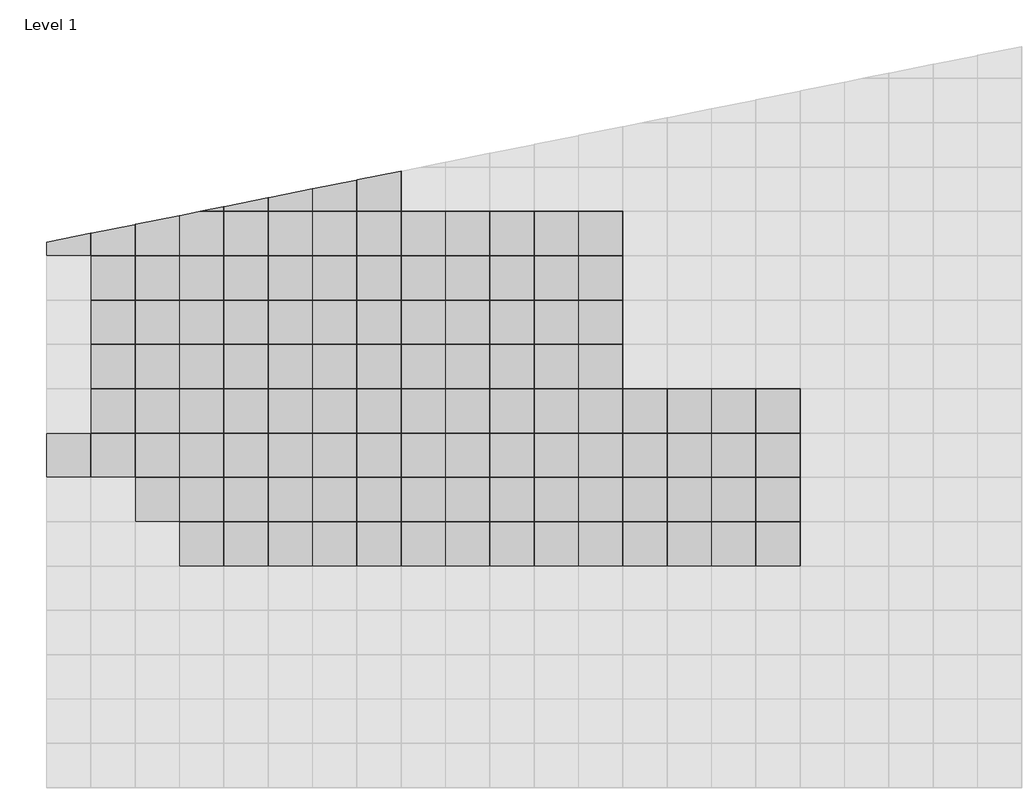
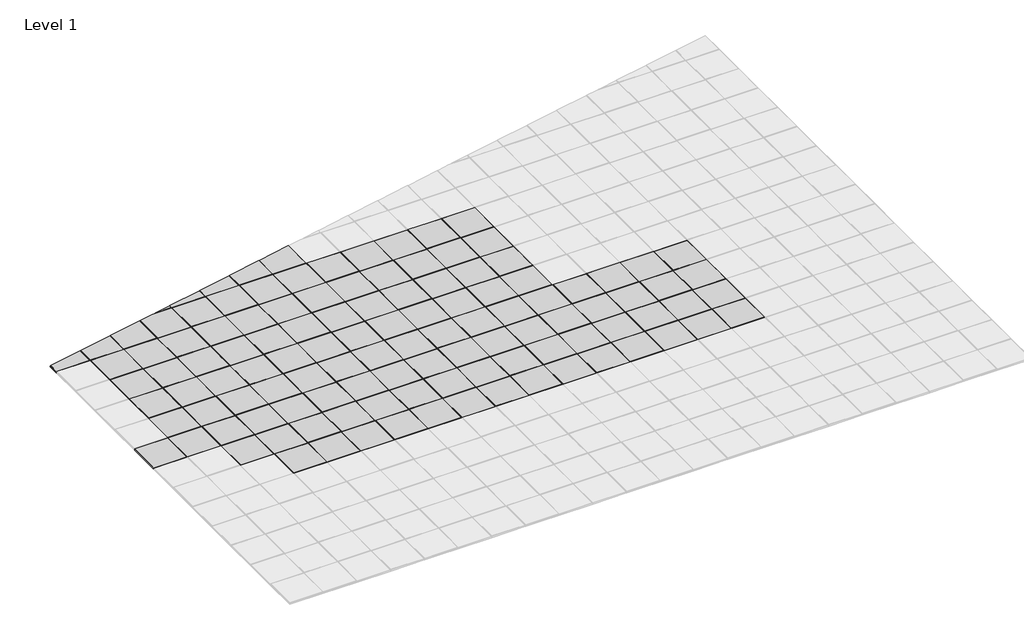
# One storey, part 5 of 18: 116 plates.
"""IFC4 building model written with IfcOpenShell, lengths in millimetres."""

import ifcopenshell
import ifcopenshell.guid

model = None  # the IFC model being written
_history = None  # IfcOwnerHistory: only IFC2X3 demands one
_inside = {}  # id of a spatial element -> (the spatial element, [elements in it])
_under = {}  # id of a project, library or spatial element -> (it, [spatial elements below it])
_declared = {}  # id of a project -> (the project, [libraries it declares])
_typed = {}  # id of a type object -> (the type object, [elements of that type])
_made_of = {}  # id of a material, layer set ... -> (it, [elements and type objects made of it])


def new_model(schema):
    """Start an empty IFC model of exactly this schema.

    Asked for "IFC4X3", IfcOpenShell would pick the latest addendum, in which some entities
    have other attributes; the version numbers below select the first issue.
    IFC2X3 requires an IfcOwnerHistory on every rooted entity: one is made here for all.
    """
    global model, _history
    if schema == "IFC4X3":
        model = ifcopenshell.file(schema_version=(4, 3, 0, 0))
    else:
        model = ifcopenshell.file(schema=schema)
    _inside.clear()
    _under.clear()
    _declared.clear()
    _typed.clear()
    _made_of.clear()
    _history = None
    if model.schema == "IFC2X3":
        org = make("IfcOrganization", Name="unknown")
        user = make(
            "IfcPersonAndOrganization",
            ThePerson=make("IfcPerson", FamilyName="unknown"),
            TheOrganization=org,
        )
        app = make(
            "IfcApplication",
            ApplicationDeveloper=org,
            Version="unknown",
            ApplicationFullName="unknown",
            ApplicationIdentifier="unknown",
        )
        _history = make(
            "IfcOwnerHistory",
            OwningUser=user,
            OwningApplication=app,
            ChangeAction="ADDED",
            CreationDate=0,
        )
    return model


def make(cls, **values):
    """One entity of the class cls with the attributes given. An attribute that is None is left unset."""
    return model.create_entity(
        cls, **{name: value for name, value in values.items() if value is not None}
    )


def rooted(cls, **values):
    """An entity with a GlobalId (a new one), such as an element, a storey or a relation."""
    return make(cls, GlobalId=ifcopenshell.guid.new(), OwnerHistory=_history, **values)


def si_unit(unit_type, name, prefix=None):
    """IfcSIUnit, for example si_unit("LENGTHUNIT", "METRE", prefix="MILLI")."""
    return make("IfcSIUnit", UnitType=unit_type, Prefix=prefix, Name=name)


def assignment(units):
    """IfcUnitAssignment: the units of a project."""
    return None if units is None else make("IfcUnitAssignment", Units=units)


def point(xyz):
    """IfcCartesianPoint."""
    return None if xyz is None else make("IfcCartesianPoint", Coordinates=xyz)


def direction(xyz):
    """IfcDirection."""
    return None if xyz is None else make("IfcDirection", DirectionRatios=xyz)


def frame(location, z_axis=None, x_axis=None):
    """IfcAxis2Placement3D, a coordinate frame: its origin and axes. An axis left out is left unset."""
    return make(
        "IfcAxis2Placement3D",
        Location=point(location),
        Axis=direction(z_axis),
        RefDirection=direction(x_axis),
    )


def origin():
    """The frame at (0, 0, 0) with its axes left unset."""
    return frame((0.0, 0.0, 0.0))


def origin_with_axes():
    """The frame at (0, 0, 0) with the z axis (0, 0, 1) and the x axis (1, 0, 0) written out."""
    return frame((0.0, 0.0, 0.0), z_axis=(0.0, 0.0, 1.0), x_axis=(1.0, 0.0, 0.0))


def place(relative_to, where):
    """IfcLocalPlacement: puts the frame where relative to a parent placement (None: the world)."""
    return make(
        "IfcLocalPlacement", PlacementRelTo=relative_to, RelativePlacement=where
    )


def context(
    kind, dimensions, precision=None, world=None, true_north=None, identifier=None
):
    """IfcGeometricRepresentationContext, for example the 3D "Model" context."""
    return make(
        "IfcGeometricRepresentationContext",
        ContextIdentifier=identifier,
        ContextType=kind,
        CoordinateSpaceDimension=dimensions,
        Precision=precision,
        WorldCoordinateSystem=world,
        TrueNorth=true_north,
    )


def project(units=None, contexts=None):
    """IfcProject with its units and contexts."""
    return rooted(
        "IfcProject",
        Name="project",
        RepresentationContexts=contexts,
        UnitsInContext=assignment(units),
    )


def spatial(cls, under=None, at=None, **own):
    """A site, building, storey or space (cls), placed at a placement, below another one or the project."""
    s = rooted(cls, ObjectPlacement=at, **own)
    if under is not None:
        _under.setdefault(under.id(), (under, []))[1].append(s)
    return s


def polyline(points):
    """IfcPolyline through the points."""
    return make("IfcPolyline", Points=[point(p) for p in points])


def outline(outer, holes=None, kind="AREA"):
    """IfcArbitraryClosedProfileDef: a profile drawn as a closed curve; with holes, ...WithVoids."""
    if holes is None:
        return make("IfcArbitraryClosedProfileDef", ProfileType=kind, OuterCurve=outer)
    return make(
        "IfcArbitraryProfileDefWithVoids",
        ProfileType=kind,
        OuterCurve=outer,
        InnerCurves=holes,
    )


def extrude(swept, where, along, depth):
    """IfcExtrudedAreaSolid: the profile swept, set in the frame where, extruded along a direction by depth."""
    return make(
        "IfcExtrudedAreaSolid",
        SweptArea=swept,
        Position=where,
        ExtrudedDirection=direction(along),
        Depth=depth,
    )


def shape(context_of_items, identifier, shape_type, items):
    """IfcShapeRepresentation: the items that make up one representation, for example the "Body"."""
    return make(
        "IfcShapeRepresentation",
        ContextOfItems=context_of_items,
        RepresentationIdentifier=identifier,
        RepresentationType=shape_type,
        Items=items,
    )


def source(mapping_origin, context_of_items, identifier, shape_type, items):
    """IfcRepresentationMap: a shape defined once, which mapped items show again and again."""
    return make(
        "IfcRepresentationMap",
        MappingOrigin=mapping_origin,
        MappedRepresentation=shape(context_of_items, identifier, shape_type, items),
    )


def transform(
    local_origin,
    x_axis=None,
    y_axis=None,
    z_axis=None,
    scale=None,
    scale2=None,
    scale3=None,
    uniform=True,
):
    """IfcCartesianTransformationOperator3D, or its non-uniform kind. x_axis, y_axis, z_axis: its Axis1, 2, 3."""
    if uniform:
        return make(
            "IfcCartesianTransformationOperator3D",
            Axis1=direction(x_axis),
            Axis2=direction(y_axis),
            LocalOrigin=point(local_origin),
            Scale=scale,
            Axis3=direction(z_axis),
        )
    return make(
        "IfcCartesianTransformationOperator3DnonUniform",
        Axis1=direction(x_axis),
        Axis2=direction(y_axis),
        LocalOrigin=point(local_origin),
        Scale=scale,
        Axis3=direction(z_axis),
        Scale2=scale2,
        Scale3=scale3,
    )


def mapped(mapping_source, mapping_target):
    """IfcMappedItem: shows the shape of a source again, moved by a transform."""
    return make(
        "IfcMappedItem", MappingSource=mapping_source, MappingTarget=mapping_target
    )


def made_of(thing, what):
    """Note that an element or type object is made of a material, layer set ...; save() writes the relation."""
    if what is not None:
        _made_of.setdefault(what.id(), (what, []))[1].append(thing)
    return thing


def element(
    cls,
    number,
    at=None,
    inside=None,
    cuts=None,
    type_object=None,
    material=None,
    context=None,
    identifier="Body",
    shape_type=None,
    held_by="IfcProductDefinitionShape",
    body=None,
    shapes=None,
    **own,
):
    """One element of the class cls, such as IfcWall. Its Tag is "e" and its number.

    at: its placement. inside: the storey or other place that contains it. cuts: it is an
    opening in that element (IfcRelVoidsElement). A single representation is given by context,
    identifier, shape_type and body (its items); several are given by shapes. held_by: the class
    of the entity that holds the representations. save() writes the other relations.
    """
    e = rooted(cls, Tag="e%d" % number, ObjectPlacement=at, **own)
    if body is not None:
        shapes = [shape(context, identifier, shape_type, body)]
    if shapes is not None:
        e.Representation = make(held_by, Representations=shapes)
    if inside is not None:
        _inside.setdefault(inside.id(), (inside, []))[1].append(e)
    if cuts is not None:
        rooted(
            "IfcRelVoidsElement", RelatingBuildingElement=cuts, RelatedOpeningElement=e
        )
    if type_object is not None:
        _typed.setdefault(type_object.id(), (type_object, []))[1].append(e)
    return made_of(e, material)


def aggregate(whole, parts):
    """IfcRelAggregates: a whole, such as a stair, and the parts it consists of."""
    return rooted("IfcRelAggregates", RelatingObject=whole, RelatedObjects=parts)


def save(model, path):
    """Write the relations noted so far, then the file.

    IfcRelAggregates (storeys below a building ...), IfcRelContainedInSpatialStructure (elements
    in a storey), IfcRelDefinesByType, IfcRelAssociatesMaterial and IfcRelDeclares: one each for
    every whole, place, type object, material and project.
    """
    for whole, parts in _under.values():
        aggregate(whole, parts)
    for where, things in _inside.values():
        rooted(
            "IfcRelContainedInSpatialStructure",
            RelatedElements=things,
            RelatingStructure=where,
        )
    for kind, things in _typed.values():
        rooted("IfcRelDefinesByType", RelatedObjects=things, RelatingType=kind)
    for what, things in _made_of.values():
        rooted("IfcRelAssociatesMaterial", RelatedObjects=things, RelatingMaterial=what)
    for by, libraries in _declared.values():
        rooted("IfcRelDeclares", RelatingContext=by, RelatedDefinitions=libraries)
    model.write(path)


def type_1_8eb2385c(model_context):
    return source(origin(), model_context, "Body", "SweptSolid", [
        extrude(outline(polyline([(1000.0, 500.0), (500.0, 500.0), (500.0, 1000.0), (1000.0, 1000.0), (1000.0, 500.0)]), holes=[polyline([(995.0, 995.0), (505.0, 995.0), (505.0, 505.0), (995.0, 505.0), (995.0, 995.0)])]), origin_with_axes(), (0.0, 0.0, 1.0), 18.0),
        extrude(outline(polyline([(505.0, 995.0), (995.0, 995.0), (995.0, 505.0), (505.0, 505.0), (505.0, 995.0)])), origin_with_axes(), (0.0, 0.0, 1.0), 20.0),
    ])


model = new_model("IFC4")

# Units and contexts
model_context = context("Model", 3, world=origin())
ifc_project = project(units=[si_unit("LENGTHUNIT", "METRE", prefix="MILLI")], contexts=[model_context])

# Site, building, storey
site = spatial("IfcSite", under=ifc_project)
building = spatial("IfcBuilding", under=site)
storey = spatial("IfcBuildingStorey", under=building, Name="Level 1", Elevation=0.0)

# Plates
placement = place(None, origin())
element("IfcPlate", 1, ObjectType="00_CPA_tegel : Type 1", at=placement, inside=storey, context=model_context, shape_type="SweptSolid", body=[
    extrude(outline(polyline([(4011.2147669, 18087.7016515), (4501.2147669, 18087.7016515), (4501.2147669, 17597.7016515), (4011.2147669, 17597.7016515), (4011.2147669, 18087.7016515)])), origin_with_axes(), (0.0, 0.0, 1.0), 20.0),
    extrude(outline(polyline([(4506.2147669, 17592.7016515), (4006.2147669, 17592.7016515), (4006.2147669, 18092.7016515), (4506.2147669, 18092.7016515), (4506.2147669, 17592.7016515)]), holes=[polyline([(4501.2147669, 18087.7016515), (4011.2147669, 18087.7016515), (4011.2147669, 17597.7016515), (4501.2147669, 17597.7016515), (4501.2147669, 18087.7016515)])]), origin_with_axes(), (0.0, 0.0, 1.0), 18.0),
])
element("IfcPlate", 2, ObjectType="00_CPA_tegel : Type 1", at=placement, inside=storey, context=model_context, shape_type="SweptSolid", body=[
    extrude(outline(polyline([(4511.2147669, 18087.7016515), (5001.2147669, 18087.7016515), (5001.2147669, 17597.7016515), (4511.2147669, 17597.7016515), (4511.2147669, 18087.7016515)])), origin_with_axes(), (0.0, 0.0, 1.0), 20.0),
    extrude(outline(polyline([(5006.2147669, 17592.7016515), (4506.2147669, 17592.7016515), (4506.2147669, 18092.7016515), (5006.2147669, 18092.7016515), (5006.2147669, 17592.7016515)]), holes=[polyline([(5001.2147669, 18087.7016515), (4511.2147669, 18087.7016515), (4511.2147669, 17597.7016515), (5001.2147669, 17597.7016515), (5001.2147669, 18087.7016515)])]), origin_with_axes(), (0.0, 0.0, 1.0), 18.0),
])
element("IfcPlate", 3, ObjectType="00_CPA_tegel : Type 1", at=placement, inside=storey, context=model_context, shape_type="SweptSolid", body=[
    extrude(outline(polyline([(6511.2147669, 18587.7016515), (7001.2147669, 18587.7016515), (7001.2147669, 18097.7016515), (6511.2147669, 18097.7016515), (6511.2147669, 18587.7016515)])), origin_with_axes(), (0.0, 0.0, 1.0), 20.0),
    extrude(outline(polyline([(7006.2147669, 18092.7016515), (6506.2147669, 18092.7016515), (6506.2147669, 18592.7016515), (7006.2147669, 18592.7016515), (7006.2147669, 18092.7016515)]), holes=[polyline([(7001.2147669, 18587.7016515), (6511.2147669, 18587.7016515), (6511.2147669, 18097.7016515), (7001.2147669, 18097.7016515), (7001.2147669, 18587.7016515)])]), origin_with_axes(), (0.0, 0.0, 1.0), 18.0),
])
element("IfcPlate", 4, ObjectType="00_CPA_tegel : Type 1", at=placement, inside=storey, context=model_context, shape_type="SweptSolid", body=[
    extrude(outline(polyline([(8511.2147669, 19087.7016515), (9001.2147669, 19087.7016515), (9001.2147669, 18597.7016515), (8511.2147669, 18597.7016515), (8511.2147669, 19087.7016515)])), origin_with_axes(), (0.0, 0.0, 1.0), 20.0),
    extrude(outline(polyline([(9006.2147669, 18592.7016515), (8506.2147669, 18592.7016515), (8506.2147669, 19092.7016515), (9006.2147669, 19092.7016515), (9006.2147669, 18592.7016515)]), holes=[polyline([(9001.2147669, 19087.7016515), (8511.2147669, 19087.7016515), (8511.2147669, 18597.7016515), (9001.2147669, 18597.7016515), (9001.2147669, 19087.7016515)])]), origin_with_axes(), (0.0, 0.0, 1.0), 18.0),
])
element("IfcPlate", 5, ObjectType="00_CPA_tegel : Type 1", at=placement, inside=storey, context=model_context, shape_type="SweptSolid", body=[
    extrude(outline(polyline([(4501.2147669, 20097.7016515), (4011.2147669, 20097.7016515), (4011.2147669, 20245.5184604), (4501.2147669, 20343.870772), (4501.2147669, 20097.7016515)])), origin_with_axes(), (0.0, 0.0, 1.0), 20.0),
    extrude(outline(polyline([(4506.2147669, 20092.7016515), (4006.2147669, 20092.7016515), (4006.2147669, 20244.5148654), (4011.2147669, 20245.5184604), (4011.2147669, 20097.7016515), (4501.2147669, 20097.7016515), (4501.2147669, 20343.870772), (4506.2147669, 20344.874367), (4506.2147669, 20092.7016515)])), origin_with_axes(), (0.0, 0.0, 1.0), 18.0),
])
element("IfcPlate", 6, ObjectType="00_CPA_tegel : Type 1", at=placement, inside=storey, context=model_context, shape_type="SweptSolid", body=[
    extrude(outline(polyline([(5001.2147669, 20097.7016515), (4511.2147669, 20097.7016515), (4511.2147669, 20345.8779621), (5001.2147669, 20444.2302737), (5001.2147669, 20097.7016515)])), origin_with_axes(), (0.0, 0.0, 1.0), 20.0),
    extrude(outline(polyline([(5006.2147669, 20092.7016515), (4506.2147669, 20092.7016515), (4506.2147669, 20344.874367), (4511.2147669, 20345.8779621), (4511.2147669, 20097.7016515), (5001.2147669, 20097.7016515), (5001.2147669, 20444.2302737), (5006.2147669, 20445.2338687), (5006.2147669, 20092.7016515)])), origin_with_axes(), (0.0, 0.0, 1.0), 18.0),
])
element("IfcPlate", 7, ObjectType="00_CPA_tegel : Type 1", at=placement, inside=storey, context=model_context, shape_type="SweptSolid", body=[
    extrude(outline(polyline([(5501.2147669, 20097.7016515), (5011.2147669, 20097.7016515), (5011.2147669, 20446.2374637), (5501.2147669, 20544.5897754), (5501.2147669, 20097.7016515)])), origin_with_axes(), (0.0, 0.0, 1.0), 20.0),
    extrude(outline(polyline([(5506.2147669, 20092.7016515), (5006.2147669, 20092.7016515), (5006.2147669, 20445.2338687), (5011.2147669, 20446.2374637), (5011.2147669, 20097.7016515), (5501.2147669, 20097.7016515), (5501.2147669, 20544.5897754), (5506.2147669, 20545.5933704), (5506.2147669, 20092.7016515)])), origin_with_axes(), (0.0, 0.0, 1.0), 18.0),
])
element("IfcPlate", 8, ObjectType="00_CPA_tegel : Type 1", at=placement, inside=storey, context=model_context, shape_type="SweptSolid", body=[
    extrude(outline(polyline([(6001.2147669, 20097.7016515), (5511.2147669, 20097.7016515), (5511.2147669, 20546.5969654), (5716.0019838, 20587.7016515), (6001.2147669, 20587.7016515), (6001.2147669, 20097.7016515)])), origin_with_axes(), (0.0, 0.0, 1.0), 20.0),
    extrude(outline(polyline([(6006.2147669, 20092.7016515), (5506.2147669, 20092.7016515), (5506.2147669, 20545.5933704), (5511.2147669, 20546.5969654), (5511.2147669, 20097.7016515), (6001.2147669, 20097.7016515), (6001.2147669, 20587.7016515), (5716.0019838, 20587.7016515), (5740.9124303, 20592.7016515), (6006.2147669, 20592.7016515), (6006.2147669, 20092.7016515)])), origin_with_axes(), (0.0, 0.0, 1.0), 18.0),
])
element("IfcPlate", 9, ObjectType="00_CPA_tegel : Type 1", at=placement, inside=storey, context=model_context, shape_type="SweptSolid", body=[
    extrude(outline(polyline([(6001.2147669, 20597.7016515), (5765.8228768, 20597.7016515), (6001.2147669, 20644.9492771), (6001.2147669, 20597.7016515)])), origin_with_axes(), (0.0, 0.0, 1.0), 20.0),
    extrude(outline(polyline([(6006.2147669, 20592.7016515), (5740.9124303, 20592.7016515), (5765.8228768, 20597.7016515), (6001.2147669, 20597.7016515), (6001.2147669, 20644.9492771), (6006.2147669, 20645.9528721), (6006.2147669, 20592.7016515)])), origin_with_axes(), (0.0, 0.0, 1.0), 18.0),
])
element("IfcPlate", 10, ObjectType="00_CPA_tegel : Type 1", at=placement, inside=storey, context=model_context, shape_type="SweptSolid", body=[
    extrude(outline(polyline([(6501.2147669, 20597.7016515), (6011.2147669, 20597.7016515), (6011.2147669, 20646.9564671), (6501.2147669, 20745.3087788), (6501.2147669, 20597.7016515)])), origin_with_axes(), (0.0, 0.0, 1.0), 20.0),
    extrude(outline(polyline([(6506.2147669, 20592.7016515), (6006.2147669, 20592.7016515), (6006.2147669, 20645.9528721), (6011.2147669, 20646.9564671), (6011.2147669, 20597.7016515), (6501.2147669, 20597.7016515), (6501.2147669, 20745.3087788), (6506.2147669, 20746.3123738), (6506.2147669, 20592.7016515)])), origin_with_axes(), (0.0, 0.0, 1.0), 18.0),
])
element("IfcPlate", 11, ObjectType="00_CPA_tegel : Type 1", at=placement, inside=storey, context=model_context, shape_type="SweptSolid", body=[
    extrude(outline(polyline([(7001.2147669, 20597.7016515), (6511.2147669, 20597.7016515), (6511.2147669, 20747.3159688), (7001.2147669, 20845.6682804), (7001.2147669, 20597.7016515)])), origin_with_axes(), (0.0, 0.0, 1.0), 20.0),
    extrude(outline(polyline([(7006.2147669, 20592.7016515), (6506.2147669, 20592.7016515), (6506.2147669, 20746.3123738), (6511.2147669, 20747.3159688), (6511.2147669, 20597.7016515), (7001.2147669, 20597.7016515), (7001.2147669, 20845.6682804), (7006.2147669, 20846.6718755), (7006.2147669, 20592.7016515)])), origin_with_axes(), (0.0, 0.0, 1.0), 18.0),
])
element("IfcPlate", 12, ObjectType="00_CPA_tegel : Type 1", at=placement, inside=storey, context=model_context, shape_type="SweptSolid", body=[
    extrude(outline(polyline([(7501.2147669, 20597.7016515), (7011.2147669, 20597.7016515), (7011.2147669, 20847.6754705), (7501.2147669, 20946.0277821), (7501.2147669, 20597.7016515)])), origin_with_axes(), (0.0, 0.0, 1.0), 20.0),
    extrude(outline(polyline([(7506.2147669, 20592.7016515), (7006.2147669, 20592.7016515), (7006.2147669, 20846.6718755), (7011.2147669, 20847.6754705), (7011.2147669, 20597.7016515), (7501.2147669, 20597.7016515), (7501.2147669, 20946.0277821), (7506.2147669, 20947.0313772), (7506.2147669, 20592.7016515)])), origin_with_axes(), (0.0, 0.0, 1.0), 18.0),
])
element("IfcPlate", 13, ObjectType="00_CPA_tegel : Type 1", at=placement, inside=storey, context=model_context, shape_type="SweptSolid", body=[
    extrude(outline(polyline([(8001.2147669, 20597.7016515), (7511.2147669, 20597.7016515), (7511.2147669, 20948.0349722), (8001.2147669, 21046.3872838), (8001.2147669, 20597.7016515)])), origin_with_axes(), (0.0, 0.0, 1.0), 20.0),
    extrude(outline(polyline([(8006.2147669, 20592.7016515), (7506.2147669, 20592.7016515), (7506.2147669, 20947.0313772), (7511.2147669, 20948.0349722), (7511.2147669, 20597.7016515), (8001.2147669, 20597.7016515), (8001.2147669, 21046.3872838), (8006.2147669, 21047.3908788), (8006.2147669, 20592.7016515)])), origin_with_axes(), (0.0, 0.0, 1.0), 18.0),
])
type_1_shape = type_1_8eb2385c(model_context)
element("IfcPlate", 14, ObjectType="00_CPA_tegel : Type 1", at=placement, inside=storey, context=model_context, shape_type="MappedRepresentation", body=[
    mapped(type_1_shape, transform((9006.2147669, 16092.7016515, 0.0), x_axis=(1.0000000000000002, 0.0, 0.0), y_axis=(0.0, 1.0000000000000002, 0.0), z_axis=(0.0, 0.0, 1.0))),
])
element("IfcPlate", 15, ObjectType="00_CPA_tegel : Type 1", at=placement, inside=storey, context=model_context, shape_type="MappedRepresentation", body=[
    mapped(type_1_shape, transform((9506.2147669, 16092.7016515, 0.0), x_axis=(1.0000000000000002, 0.0, 0.0), y_axis=(0.0, 1.0000000000000002, 0.0), z_axis=(0.0, 0.0, 1.0))),
])
element("IfcPlate", 16, ObjectType="00_CPA_tegel : Type 1", at=placement, inside=storey, context=model_context, shape_type="MappedRepresentation", body=[
    mapped(type_1_shape, transform((6006.2147669, 16092.7016515, 0.0), x_axis=(1.0000000000000002, 0.0, 0.0), y_axis=(0.0, 1.0000000000000002, 0.0), z_axis=(0.0, 0.0, 1.0))),
])
element("IfcPlate", 17, ObjectType="00_CPA_tegel : Type 1", at=placement, inside=storey, context=model_context, shape_type="MappedRepresentation", body=[
    mapped(type_1_shape, transform((6506.2147669, 16092.7016515, 0.0), x_axis=(1.0000000000000002, 0.0, 0.0), y_axis=(0.0, 1.0000000000000002, 0.0), z_axis=(0.0, 0.0, 1.0))),
])
element("IfcPlate", 18, ObjectType="00_CPA_tegel : Type 1", at=placement, inside=storey, context=model_context, shape_type="MappedRepresentation", body=[
    mapped(type_1_shape, transform((7006.2147669, 16092.7016515, 0.0), x_axis=(1.0000000000000002, 0.0, 0.0), y_axis=(0.0, 1.0000000000000002, 0.0), z_axis=(0.0, 0.0, 1.0))),
])
element("IfcPlate", 19, ObjectType="00_CPA_tegel : Type 1", at=placement, inside=storey, context=model_context, shape_type="MappedRepresentation", body=[
    mapped(type_1_shape, transform((7506.2147669, 16092.7016515, 0.0), x_axis=(1.0000000000000002, 0.0, 0.0), y_axis=(0.0, 1.0000000000000002, 0.0), z_axis=(0.0, 0.0, 1.0))),
])
element("IfcPlate", 20, ObjectType="00_CPA_tegel : Type 1", at=placement, inside=storey, context=model_context, shape_type="MappedRepresentation", body=[
    mapped(type_1_shape, transform((8006.2147669, 16092.7016515, 0.0), x_axis=(1.0000000000000002, 0.0, 0.0), y_axis=(0.0, 1.0000000000000002, 0.0), z_axis=(0.0, 0.0, 1.0))),
])
element("IfcPlate", 21, ObjectType="00_CPA_tegel : Type 1", at=placement, inside=storey, context=model_context, shape_type="MappedRepresentation", body=[
    mapped(type_1_shape, transform((8506.2147669, 16092.7016515, 0.0), x_axis=(1.0000000000000002, 0.0, 0.0), y_axis=(0.0, 1.0000000000000002, 0.0), z_axis=(0.0, 0.0, 1.0))),
])
element("IfcPlate", 22, ObjectType="00_CPA_tegel : Type 1", at=placement, inside=storey, context=model_context, shape_type="MappedRepresentation", body=[
    mapped(type_1_shape, transform((8506.2147669, 16592.7016515, 0.0), x_axis=(1.0000000000000002, 0.0, 0.0), y_axis=(0.0, 1.0000000000000002, 0.0), z_axis=(0.0, 0.0, 1.0))),
])
element("IfcPlate", 23, ObjectType="00_CPA_tegel : Type 1", at=placement, inside=storey, context=model_context, shape_type="MappedRepresentation", body=[
    mapped(type_1_shape, transform((9006.2147669, 16592.7016515, 0.0), x_axis=(1.0000000000000002, 0.0, 0.0), y_axis=(0.0, 1.0000000000000002, 0.0), z_axis=(0.0, 0.0, 1.0))),
])
element("IfcPlate", 24, ObjectType="00_CPA_tegel : Type 1", at=placement, inside=storey, context=model_context, shape_type="MappedRepresentation", body=[
    mapped(type_1_shape, transform((9506.2147669, 16592.7016515, 0.0), x_axis=(1.0000000000000002, 0.0, 0.0), y_axis=(0.0, 1.0000000000000002, 0.0), z_axis=(0.0, 0.0, 1.0))),
])
element("IfcPlate", 25, ObjectType="00_CPA_tegel : Type 1", at=placement, inside=storey, context=model_context, shape_type="MappedRepresentation", body=[
    mapped(type_1_shape, transform((5506.2147669, 16092.7016515, 0.0), x_axis=(1.0000000000000002, 0.0, 0.0), y_axis=(0.0, 1.0000000000000002, 0.0), z_axis=(0.0, 0.0, 1.0))),
])
element("IfcPlate", 26, ObjectType="00_CPA_tegel : Type 1", at=placement, inside=storey, context=model_context, shape_type="MappedRepresentation", body=[
    mapped(type_1_shape, transform((7506.2147669, 16592.7016515, 0.0), x_axis=(1.0000000000000002, 0.0, 0.0), y_axis=(0.0, 1.0000000000000002, 0.0), z_axis=(0.0, 0.0, 1.0))),
])
element("IfcPlate", 27, ObjectType="00_CPA_tegel : Type 1", at=placement, inside=storey, context=model_context, shape_type="MappedRepresentation", body=[
    mapped(type_1_shape, transform((8006.2147669, 16592.7016515, 0.0), x_axis=(1.0000000000000002, 0.0, 0.0), y_axis=(0.0, 1.0000000000000002, 0.0), z_axis=(0.0, 0.0, 1.0))),
])
element("IfcPlate", 28, ObjectType="00_CPA_tegel : Type 1", at=placement, inside=storey, context=model_context, shape_type="MappedRepresentation", body=[
    mapped(type_1_shape, transform((10006.2147669, 16592.7016515, 0.0), x_axis=(1.0000000000000002, 0.0, 0.0), y_axis=(0.0, 1.0000000000000002, 0.0), z_axis=(0.0, 0.0, 1.0))),
])
element("IfcPlate", 29, ObjectType="00_CPA_tegel : Type 1", at=placement, inside=storey, context=model_context, shape_type="MappedRepresentation", body=[
    mapped(type_1_shape, transform((10006.2147669, 17092.7016515, 0.0), x_axis=(1.0000000000000002, 0.0, 0.0), y_axis=(0.0, 1.0000000000000002, 0.0), z_axis=(0.0, 0.0, 1.0))),
])
element("IfcPlate", 30, ObjectType="00_CPA_tegel : Type 1", at=placement, inside=storey, context=model_context, shape_type="MappedRepresentation", body=[
    mapped(type_1_shape, transform((5006.2147669, 16092.7016515, 0.0), x_axis=(1.0000000000000002, 0.0, 0.0), y_axis=(0.0, 1.0000000000000002, 0.0), z_axis=(0.0, 0.0, 1.0))),
])
element("IfcPlate", 31, ObjectType="00_CPA_tegel : Type 1", at=placement, inside=storey, context=model_context, shape_type="MappedRepresentation", body=[
    mapped(type_1_shape, transform((10006.2147669, 16092.7016515, 0.0), x_axis=(1.0000000000000002, 0.0, 0.0), y_axis=(0.0, 1.0000000000000002, 0.0), z_axis=(0.0, 0.0, 1.0))),
])
element("IfcPlate", 32, ObjectType="00_CPA_tegel : Type 1", at=placement, inside=storey, context=model_context, shape_type="MappedRepresentation", body=[
    mapped(type_1_shape, transform((9506.2147669, 17092.7016515, 0.0), x_axis=(1.0000000000000002, 0.0, 0.0), y_axis=(0.0, 1.0000000000000002, 0.0), z_axis=(0.0, 0.0, 1.0))),
])
element("IfcPlate", 33, ObjectType="00_CPA_tegel : Type 1", at=placement, inside=storey, context=model_context, shape_type="MappedRepresentation", body=[
    mapped(type_1_shape, transform((6006.2147669, 16592.7016515, 0.0), x_axis=(1.0000000000000002, 0.0, 0.0), y_axis=(0.0, 1.0000000000000002, 0.0), z_axis=(0.0, 0.0, 1.0))),
])
element("IfcPlate", 34, ObjectType="00_CPA_tegel : Type 1", at=placement, inside=storey, context=model_context, shape_type="MappedRepresentation", body=[
    mapped(type_1_shape, transform((6506.2147669, 16592.7016515, 0.0), x_axis=(1.0000000000000002, 0.0, 0.0), y_axis=(0.0, 1.0000000000000002, 0.0), z_axis=(0.0, 0.0, 1.0))),
])
element("IfcPlate", 35, ObjectType="00_CPA_tegel : Type 1", at=placement, inside=storey, context=model_context, shape_type="MappedRepresentation", body=[
    mapped(type_1_shape, transform((7006.2147669, 16592.7016515, 0.0), x_axis=(1.0000000000000002, 0.0, 0.0), y_axis=(0.0, 1.0000000000000002, 0.0), z_axis=(0.0, 0.0, 1.0))),
])
element("IfcPlate", 36, ObjectType="00_CPA_tegel : Type 1", at=placement, inside=storey, context=model_context, shape_type="MappedRepresentation", body=[
    mapped(type_1_shape, transform((8006.2147669, 17092.7016515, 0.0), x_axis=(1.0000000000000002, 0.0, 0.0), y_axis=(0.0, 1.0000000000000002, 0.0), z_axis=(0.0, 0.0, 1.0))),
])
element("IfcPlate", 37, ObjectType="00_CPA_tegel : Type 1", at=placement, inside=storey, context=model_context, shape_type="MappedRepresentation", body=[
    mapped(type_1_shape, transform((8506.2147669, 17092.7016515, 0.0), x_axis=(1.0000000000000002, 0.0, 0.0), y_axis=(0.0, 1.0000000000000002, 0.0), z_axis=(0.0, 0.0, 1.0))),
])
element("IfcPlate", 38, ObjectType="00_CPA_tegel : Type 1", at=placement, inside=storey, context=model_context, shape_type="MappedRepresentation", body=[
    mapped(type_1_shape, transform((9006.2147669, 17092.7016515, 0.0), x_axis=(1.0000000000000002, 0.0, 0.0), y_axis=(0.0, 1.0000000000000002, 0.0), z_axis=(0.0, 0.0, 1.0))),
])
element("IfcPlate", 39, ObjectType="00_CPA_tegel : Type 1", at=placement, inside=storey, context=model_context, shape_type="MappedRepresentation", body=[
    mapped(type_1_shape, transform((10506.2147669, 17092.7016515, 0.0), x_axis=(1.0000000000000002, 0.0, 0.0), y_axis=(0.0, 1.0000000000000002, 0.0), z_axis=(0.0, 0.0, 1.0))),
])
element("IfcPlate", 40, ObjectType="00_CPA_tegel : Type 1", at=placement, inside=storey, context=model_context, shape_type="MappedRepresentation", body=[
    mapped(type_1_shape, transform((10506.2147669, 17592.7016515, 0.0), x_axis=(1.0000000000000002, 0.0, 0.0), y_axis=(0.0, 1.0000000000000002, 0.0), z_axis=(0.0, 0.0, 1.0))),
])
element("IfcPlate", 41, ObjectType="00_CPA_tegel : Type 1", at=placement, inside=storey, context=model_context, shape_type="MappedRepresentation", body=[
    mapped(type_1_shape, transform((10506.2147669, 16092.7016515, 0.0), x_axis=(1.0000000000000002, 0.0, 0.0), y_axis=(0.0, 1.0000000000000002, 0.0), z_axis=(0.0, 0.0, 1.0))),
])
element("IfcPlate", 42, ObjectType="00_CPA_tegel : Type 1", at=placement, inside=storey, context=model_context, shape_type="MappedRepresentation", body=[
    mapped(type_1_shape, transform((4506.2147669, 16592.7016515, 0.0), x_axis=(1.0000000000000002, 0.0, 0.0), y_axis=(0.0, 1.0000000000000002, 0.0), z_axis=(0.0, 0.0, 1.0))),
])
element("IfcPlate", 43, ObjectType="00_CPA_tegel : Type 1", at=placement, inside=storey, context=model_context, shape_type="MappedRepresentation", body=[
    mapped(type_1_shape, transform((5006.2147669, 16592.7016515, 0.0), x_axis=(1.0000000000000002, 0.0, 0.0), y_axis=(0.0, 1.0000000000000002, 0.0), z_axis=(0.0, 0.0, 1.0))),
])
element("IfcPlate", 44, ObjectType="00_CPA_tegel : Type 1", at=placement, inside=storey, context=model_context, shape_type="MappedRepresentation", body=[
    mapped(type_1_shape, transform((5506.2147669, 16592.7016515, 0.0), x_axis=(1.0000000000000002, 0.0, 0.0), y_axis=(0.0, 1.0000000000000002, 0.0), z_axis=(0.0, 0.0, 1.0))),
])
element("IfcPlate", 45, ObjectType="00_CPA_tegel : Type 1", at=placement, inside=storey, context=model_context, shape_type="MappedRepresentation", body=[
    mapped(type_1_shape, transform((10506.2147669, 16592.7016515, 0.0), x_axis=(1.0000000000000002, 0.0, 0.0), y_axis=(0.0, 1.0000000000000002, 0.0), z_axis=(0.0, 0.0, 1.0))),
])
element("IfcPlate", 46, ObjectType="00_CPA_tegel : Type 1", at=placement, inside=storey, context=model_context, shape_type="MappedRepresentation", body=[
    mapped(type_1_shape, transform((11006.2147669, 16592.7016515, 0.0), x_axis=(1.0000000000000002, 0.0, 0.0), y_axis=(0.0, 1.0000000000000002, 0.0), z_axis=(0.0, 0.0, 1.0))),
])
element("IfcPlate", 47, ObjectType="00_CPA_tegel : Type 1", at=placement, inside=storey, context=model_context, shape_type="MappedRepresentation", body=[
    mapped(type_1_shape, transform((5506.2147669, 17092.7016515, 0.0), x_axis=(1.0000000000000002, 0.0, 0.0), y_axis=(0.0, 1.0000000000000002, 0.0), z_axis=(0.0, 0.0, 1.0))),
])
element("IfcPlate", 48, ObjectType="00_CPA_tegel : Type 1", at=placement, inside=storey, context=model_context, shape_type="MappedRepresentation", body=[
    mapped(type_1_shape, transform((6006.2147669, 17092.7016515, 0.0), x_axis=(1.0000000000000002, 0.0, 0.0), y_axis=(0.0, 1.0000000000000002, 0.0), z_axis=(0.0, 0.0, 1.0))),
])
element("IfcPlate", 49, ObjectType="00_CPA_tegel : Type 1", at=placement, inside=storey, context=model_context, shape_type="MappedRepresentation", body=[
    mapped(type_1_shape, transform((6506.2147669, 17092.7016515, 0.0), x_axis=(1.0000000000000002, 0.0, 0.0), y_axis=(0.0, 1.0000000000000002, 0.0), z_axis=(0.0, 0.0, 1.0))),
])
element("IfcPlate", 50, ObjectType="00_CPA_tegel : Type 1", at=placement, inside=storey, context=model_context, shape_type="MappedRepresentation", body=[
    mapped(type_1_shape, transform((7006.2147669, 17092.7016515, 0.0), x_axis=(1.0000000000000002, 0.0, 0.0), y_axis=(0.0, 1.0000000000000002, 0.0), z_axis=(0.0, 0.0, 1.0))),
])
element("IfcPlate", 51, ObjectType="00_CPA_tegel : Type 1", at=placement, inside=storey, context=model_context, shape_type="MappedRepresentation", body=[
    mapped(type_1_shape, transform((7506.2147669, 17092.7016515, 0.0), x_axis=(1.0000000000000002, 0.0, 0.0), y_axis=(0.0, 1.0000000000000002, 0.0), z_axis=(0.0, 0.0, 1.0))),
])
element("IfcPlate", 52, ObjectType="00_CPA_tegel : Type 1", at=placement, inside=storey, context=model_context, shape_type="MappedRepresentation", body=[
    mapped(type_1_shape, transform((11006.2147669, 17092.7016515, 0.0), x_axis=(1.0000000000000002, 0.0, 0.0), y_axis=(0.0, 1.0000000000000002, 0.0), z_axis=(0.0, 0.0, 1.0))),
])
element("IfcPlate", 53, ObjectType="00_CPA_tegel : Type 1", at=placement, inside=storey, context=model_context, shape_type="MappedRepresentation", body=[
    mapped(type_1_shape, transform((7506.2147669, 17592.7016515, 0.0), x_axis=(1.0000000000000002, 0.0, 0.0), y_axis=(0.0, 1.0000000000000002, 0.0), z_axis=(0.0, 0.0, 1.0))),
])
element("IfcPlate", 54, ObjectType="00_CPA_tegel : Type 1", at=placement, inside=storey, context=model_context, shape_type="MappedRepresentation", body=[
    mapped(type_1_shape, transform((8006.2147669, 17592.7016515, 0.0), x_axis=(1.0000000000000002, 0.0, 0.0), y_axis=(0.0, 1.0000000000000002, 0.0), z_axis=(0.0, 0.0, 1.0))),
])
element("IfcPlate", 55, ObjectType="00_CPA_tegel : Type 1", at=placement, inside=storey, context=model_context, shape_type="MappedRepresentation", body=[
    mapped(type_1_shape, transform((8506.2147669, 17592.7016515, 0.0), x_axis=(1.0000000000000002, 0.0, 0.0), y_axis=(0.0, 1.0000000000000002, 0.0), z_axis=(0.0, 0.0, 1.0))),
])
element("IfcPlate", 56, ObjectType="00_CPA_tegel : Type 1", at=placement, inside=storey, context=model_context, shape_type="MappedRepresentation", body=[
    mapped(type_1_shape, transform((9006.2147669, 17592.7016515, 0.0), x_axis=(1.0000000000000002, 0.0, 0.0), y_axis=(0.0, 1.0000000000000002, 0.0), z_axis=(0.0, 0.0, 1.0))),
])
element("IfcPlate", 57, ObjectType="00_CPA_tegel : Type 1", at=placement, inside=storey, context=model_context, shape_type="MappedRepresentation", body=[
    mapped(type_1_shape, transform((9506.2147669, 17592.7016515, 0.0), x_axis=(1.0000000000000002, 0.0, 0.0), y_axis=(0.0, 1.0000000000000002, 0.0), z_axis=(0.0, 0.0, 1.0))),
])
element("IfcPlate", 58, ObjectType="00_CPA_tegel : Type 1", at=placement, inside=storey, context=model_context, shape_type="MappedRepresentation", body=[
    mapped(type_1_shape, transform((10006.2147669, 17592.7016515, 0.0), x_axis=(1.0000000000000002, 0.0, 0.0), y_axis=(0.0, 1.0000000000000002, 0.0), z_axis=(0.0, 0.0, 1.0))),
])
element("IfcPlate", 59, ObjectType="00_CPA_tegel : Type 1", at=placement, inside=storey, context=model_context, shape_type="MappedRepresentation", body=[
    mapped(type_1_shape, transform((11006.2147669, 17592.7016515, 0.0), x_axis=(1.0000000000000002, 0.0, 0.0), y_axis=(0.0, 1.0000000000000002, 0.0), z_axis=(0.0, 0.0, 1.0))),
])
element("IfcPlate", 60, ObjectType="00_CPA_tegel : Type 1", at=placement, inside=storey, context=model_context, shape_type="MappedRepresentation", body=[
    mapped(type_1_shape, transform((11006.2147669, 16092.7016515, 0.0), x_axis=(1.0000000000000002, 0.0, 0.0), y_axis=(0.0, 1.0000000000000002, 0.0), z_axis=(0.0, 0.0, 1.0))),
])
element("IfcPlate", 61, ObjectType="00_CPA_tegel : Type 1", at=placement, inside=storey, context=model_context, shape_type="MappedRepresentation", body=[
    mapped(type_1_shape, transform((11506.2147669, 16092.7016515, 0.0), x_axis=(1.0000000000000002, 0.0, 0.0), y_axis=(0.0, 1.0000000000000002, 0.0), z_axis=(0.0, 0.0, 1.0))),
])
element("IfcPlate", 62, ObjectType="00_CPA_tegel : Type 1", at=placement, inside=storey, context=model_context, shape_type="MappedRepresentation", body=[
    mapped(type_1_shape, transform((11506.2147669, 16592.7016515, 0.0), x_axis=(1.0000000000000002, 0.0, 0.0), y_axis=(0.0, 1.0000000000000002, 0.0), z_axis=(0.0, 0.0, 1.0))),
])
element("IfcPlate", 63, ObjectType="00_CPA_tegel : Type 1", at=placement, inside=storey, context=model_context, shape_type="MappedRepresentation", body=[
    mapped(type_1_shape, transform((4506.2147669, 17092.7016515, 0.0), x_axis=(1.0000000000000002, 0.0, 0.0), y_axis=(0.0, 1.0000000000000002, 0.0), z_axis=(0.0, 0.0, 1.0))),
])
element("IfcPlate", 64, ObjectType="00_CPA_tegel : Type 1", at=placement, inside=storey, context=model_context, shape_type="MappedRepresentation", body=[
    mapped(type_1_shape, transform((5006.2147669, 17092.7016515, 0.0), x_axis=(1.0000000000000002, 0.0, 0.0), y_axis=(0.0, 1.0000000000000002, 0.0), z_axis=(0.0, 0.0, 1.0))),
])
element("IfcPlate", 65, ObjectType="00_CPA_tegel : Type 1", at=placement, inside=storey, context=model_context, shape_type="MappedRepresentation", body=[
    mapped(type_1_shape, transform((11506.2147669, 17092.7016515, 0.0), x_axis=(1.0000000000000002, 0.0, 0.0), y_axis=(0.0, 1.0000000000000002, 0.0), z_axis=(0.0, 0.0, 1.0))),
])
element("IfcPlate", 66, ObjectType="00_CPA_tegel : Type 1", at=placement, inside=storey, context=model_context, shape_type="MappedRepresentation", body=[
    mapped(type_1_shape, transform((4006.2147669, 17592.7016515, 0.0), x_axis=(1.0000000000000002, 0.0, 0.0), y_axis=(0.0, 1.0000000000000002, 0.0), z_axis=(0.0, 0.0, 1.0))),
])
element("IfcPlate", 67, ObjectType="00_CPA_tegel : Type 1", at=placement, inside=storey, context=model_context, shape_type="MappedRepresentation", body=[
    mapped(type_1_shape, transform((4506.2147669, 17592.7016515, 0.0), x_axis=(1.0000000000000002, 0.0, 0.0), y_axis=(0.0, 1.0000000000000002, 0.0), z_axis=(0.0, 0.0, 1.0))),
])
element("IfcPlate", 68, ObjectType="00_CPA_tegel : Type 1", at=placement, inside=storey, context=model_context, shape_type="MappedRepresentation", body=[
    mapped(type_1_shape, transform((5006.2147669, 17592.7016515, 0.0), x_axis=(1.0000000000000002, 0.0, 0.0), y_axis=(0.0, 1.0000000000000002, 0.0), z_axis=(0.0, 0.0, 1.0))),
])
element("IfcPlate", 69, ObjectType="00_CPA_tegel : Type 1", at=placement, inside=storey, context=model_context, shape_type="MappedRepresentation", body=[
    mapped(type_1_shape, transform((5506.2147669, 17592.7016515, 0.0), x_axis=(1.0000000000000002, 0.0, 0.0), y_axis=(0.0, 1.0000000000000002, 0.0), z_axis=(0.0, 0.0, 1.0))),
])
element("IfcPlate", 70, ObjectType="00_CPA_tegel : Type 1", at=placement, inside=storey, context=model_context, shape_type="MappedRepresentation", body=[
    mapped(type_1_shape, transform((6506.2147669, 17592.7016515, 0.0), x_axis=(1.0000000000000002, 0.0, 0.0), y_axis=(0.0, 1.0000000000000002, 0.0), z_axis=(0.0, 0.0, 1.0))),
])
element("IfcPlate", 71, ObjectType="00_CPA_tegel : Type 1", at=placement, inside=storey, context=model_context, shape_type="MappedRepresentation", body=[
    mapped(type_1_shape, transform((7006.2147669, 17592.7016515, 0.0), x_axis=(1.0000000000000002, 0.0, 0.0), y_axis=(0.0, 1.0000000000000002, 0.0), z_axis=(0.0, 0.0, 1.0))),
])
element("IfcPlate", 72, ObjectType="00_CPA_tegel : Type 1", at=placement, inside=storey, context=model_context, shape_type="MappedRepresentation", body=[
    mapped(type_1_shape, transform((11506.2147669, 17592.7016515, 0.0), x_axis=(1.0000000000000002, 0.0, 0.0), y_axis=(0.0, 1.0000000000000002, 0.0), z_axis=(0.0, 0.0, 1.0))),
])
element("IfcPlate", 73, ObjectType="00_CPA_tegel : Type 1", at=placement, inside=storey, context=model_context, shape_type="MappedRepresentation", body=[
    mapped(type_1_shape, transform((4006.2147669, 18092.7016515, 0.0), x_axis=(1.0000000000000002, 0.0, 0.0), y_axis=(0.0, 1.0000000000000002, 0.0), z_axis=(0.0, 0.0, 1.0))),
])
element("IfcPlate", 74, ObjectType="00_CPA_tegel : Type 1", at=placement, inside=storey, context=model_context, shape_type="MappedRepresentation", body=[
    mapped(type_1_shape, transform((4506.2147669, 18092.7016515, 0.0), x_axis=(1.0000000000000002, 0.0, 0.0), y_axis=(0.0, 1.0000000000000002, 0.0), z_axis=(0.0, 0.0, 1.0))),
])
element("IfcPlate", 75, ObjectType="00_CPA_tegel : Type 1", at=placement, inside=storey, context=model_context, shape_type="MappedRepresentation", body=[
    mapped(type_1_shape, transform((5006.2147669, 18092.7016515, 0.0), x_axis=(1.0000000000000002, 0.0, 0.0), y_axis=(0.0, 1.0000000000000002, 0.0), z_axis=(0.0, 0.0, 1.0))),
])
element("IfcPlate", 76, ObjectType="00_CPA_tegel : Type 1", at=placement, inside=storey, context=model_context, shape_type="MappedRepresentation", body=[
    mapped(type_1_shape, transform((5506.2147669, 18092.7016515, 0.0), x_axis=(1.0000000000000002, 0.0, 0.0), y_axis=(0.0, 1.0000000000000002, 0.0), z_axis=(0.0, 0.0, 1.0))),
])
element("IfcPlate", 77, ObjectType="00_CPA_tegel : Type 1", at=placement, inside=storey, context=model_context, shape_type="MappedRepresentation", body=[
    mapped(type_1_shape, transform((6006.2147669, 18092.7016515, 0.0), x_axis=(1.0000000000000002, 0.0, 0.0), y_axis=(0.0, 1.0000000000000002, 0.0), z_axis=(0.0, 0.0, 1.0))),
])
element("IfcPlate", 78, ObjectType="00_CPA_tegel : Type 1", at=placement, inside=storey, context=model_context, shape_type="MappedRepresentation", body=[
    mapped(type_1_shape, transform((6506.2147669, 18092.7016515, 0.0), x_axis=(1.0000000000000002, 0.0, 0.0), y_axis=(0.0, 1.0000000000000002, 0.0), z_axis=(0.0, 0.0, 1.0))),
])
element("IfcPlate", 79, ObjectType="00_CPA_tegel : Type 1", at=placement, inside=storey, context=model_context, shape_type="MappedRepresentation", body=[
    mapped(type_1_shape, transform((7006.2147669, 18092.7016515, 0.0), x_axis=(1.0000000000000002, 0.0, 0.0), y_axis=(0.0, 1.0000000000000002, 0.0), z_axis=(0.0, 0.0, 1.0))),
])
element("IfcPlate", 80, ObjectType="00_CPA_tegel : Type 1", at=placement, inside=storey, context=model_context, shape_type="MappedRepresentation", body=[
    mapped(type_1_shape, transform((7506.2147669, 18092.7016515, 0.0), x_axis=(1.0000000000000002, 0.0, 0.0), y_axis=(0.0, 1.0000000000000002, 0.0), z_axis=(0.0, 0.0, 1.0))),
])
element("IfcPlate", 81, ObjectType="00_CPA_tegel : Type 1", at=placement, inside=storey, context=model_context, shape_type="MappedRepresentation", body=[
    mapped(type_1_shape, transform((8506.2147669, 18092.7016515, 0.0), x_axis=(1.0000000000000002, 0.0, 0.0), y_axis=(0.0, 1.0000000000000002, 0.0), z_axis=(0.0, 0.0, 1.0))),
])
element("IfcPlate", 82, ObjectType="00_CPA_tegel : Type 1", at=placement, inside=storey, context=model_context, shape_type="MappedRepresentation", body=[
    mapped(type_1_shape, transform((9006.2147669, 18092.7016515, 0.0), x_axis=(1.0000000000000002, 0.0, 0.0), y_axis=(0.0, 1.0000000000000002, 0.0), z_axis=(0.0, 0.0, 1.0))),
])
element("IfcPlate", 83, ObjectType="00_CPA_tegel : Type 1", at=placement, inside=storey, context=model_context, shape_type="MappedRepresentation", body=[
    mapped(type_1_shape, transform((9506.2147669, 18092.7016515, 0.0), x_axis=(1.0000000000000002, 0.0, 0.0), y_axis=(0.0, 1.0000000000000002, 0.0), z_axis=(0.0, 0.0, 1.0))),
])
element("IfcPlate", 84, ObjectType="00_CPA_tegel : Type 1", at=placement, inside=storey, context=model_context, shape_type="MappedRepresentation", body=[
    mapped(type_1_shape, transform((4006.2147669, 18592.7016515, 0.0), x_axis=(1.0000000000000002, 0.0, 0.0), y_axis=(0.0, 1.0000000000000002, 0.0), z_axis=(0.0, 0.0, 1.0))),
])
element("IfcPlate", 85, ObjectType="00_CPA_tegel : Type 1", at=placement, inside=storey, context=model_context, shape_type="MappedRepresentation", body=[
    mapped(type_1_shape, transform((4506.2147669, 18592.7016515, 0.0), x_axis=(1.0000000000000002, 0.0, 0.0), y_axis=(0.0, 1.0000000000000002, 0.0), z_axis=(0.0, 0.0, 1.0))),
])
element("IfcPlate", 86, ObjectType="00_CPA_tegel : Type 1", at=placement, inside=storey, context=model_context, shape_type="MappedRepresentation", body=[
    mapped(type_1_shape, transform((5006.2147669, 18592.7016515, 0.0), x_axis=(1.0000000000000002, 0.0, 0.0), y_axis=(0.0, 1.0000000000000002, 0.0), z_axis=(0.0, 0.0, 1.0))),
])
element("IfcPlate", 87, ObjectType="00_CPA_tegel : Type 1", at=placement, inside=storey, context=model_context, shape_type="MappedRepresentation", body=[
    mapped(type_1_shape, transform((5506.2147669, 18592.7016515, 0.0), x_axis=(1.0000000000000002, 0.0, 0.0), y_axis=(0.0, 1.0000000000000002, 0.0), z_axis=(0.0, 0.0, 1.0))),
])
element("IfcPlate", 88, ObjectType="00_CPA_tegel : Type 1", at=placement, inside=storey, context=model_context, shape_type="MappedRepresentation", body=[
    mapped(type_1_shape, transform((6006.2147669, 18592.7016515, 0.0), x_axis=(1.0000000000000002, 0.0, 0.0), y_axis=(0.0, 1.0000000000000002, 0.0), z_axis=(0.0, 0.0, 1.0))),
])
element("IfcPlate", 89, ObjectType="00_CPA_tegel : Type 1", at=placement, inside=storey, context=model_context, shape_type="MappedRepresentation", body=[
    mapped(type_1_shape, transform((6506.2147669, 18592.7016515, 0.0), x_axis=(1.0000000000000002, 0.0, 0.0), y_axis=(0.0, 1.0000000000000002, 0.0), z_axis=(0.0, 0.0, 1.0))),
])
element("IfcPlate", 90, ObjectType="00_CPA_tegel : Type 1", at=placement, inside=storey, context=model_context, shape_type="MappedRepresentation", body=[
    mapped(type_1_shape, transform((7006.2147669, 18592.7016515, 0.0), x_axis=(1.0000000000000002, 0.0, 0.0), y_axis=(0.0, 1.0000000000000002, 0.0), z_axis=(0.0, 0.0, 1.0))),
])
element("IfcPlate", 91, ObjectType="00_CPA_tegel : Type 1", at=placement, inside=storey, context=model_context, shape_type="MappedRepresentation", body=[
    mapped(type_1_shape, transform((7506.2147669, 18592.7016515, 0.0), x_axis=(1.0000000000000002, 0.0, 0.0), y_axis=(0.0, 1.0000000000000002, 0.0), z_axis=(0.0, 0.0, 1.0))),
])
element("IfcPlate", 92, ObjectType="00_CPA_tegel : Type 1", at=placement, inside=storey, context=model_context, shape_type="MappedRepresentation", body=[
    mapped(type_1_shape, transform((8006.2147669, 18592.7016515, 0.0), x_axis=(1.0000000000000002, 0.0, 0.0), y_axis=(0.0, 1.0000000000000002, 0.0), z_axis=(0.0, 0.0, 1.0))),
])
element("IfcPlate", 93, ObjectType="00_CPA_tegel : Type 1", at=placement, inside=storey, context=model_context, shape_type="MappedRepresentation", body=[
    mapped(type_1_shape, transform((8506.2147669, 18592.7016515, 0.0), x_axis=(1.0000000000000002, 0.0, 0.0), y_axis=(0.0, 1.0000000000000002, 0.0), z_axis=(0.0, 0.0, 1.0))),
])
element("IfcPlate", 94, ObjectType="00_CPA_tegel : Type 1", at=placement, inside=storey, context=model_context, shape_type="MappedRepresentation", body=[
    mapped(type_1_shape, transform((9006.2147669, 18592.7016515, 0.0), x_axis=(1.0000000000000002, 0.0, 0.0), y_axis=(0.0, 1.0000000000000002, 0.0), z_axis=(0.0, 0.0, 1.0))),
])
element("IfcPlate", 95, ObjectType="00_CPA_tegel : Type 1", at=placement, inside=storey, context=model_context, shape_type="MappedRepresentation", body=[
    mapped(type_1_shape, transform((9506.2147669, 18592.7016515, 0.0), x_axis=(1.0000000000000002, 0.0, 0.0), y_axis=(0.0, 1.0000000000000002, 0.0), z_axis=(0.0, 0.0, 1.0))),
])
element("IfcPlate", 96, ObjectType="00_CPA_tegel : Type 1", at=placement, inside=storey, context=model_context, shape_type="MappedRepresentation", body=[
    mapped(type_1_shape, transform((4006.2147669, 19092.7016515, 0.0), x_axis=(1.0000000000000002, 0.0, 0.0), y_axis=(0.0, 1.0000000000000002, 0.0), z_axis=(0.0, 0.0, 1.0))),
])
element("IfcPlate", 97, ObjectType="00_CPA_tegel : Type 1", at=placement, inside=storey, context=model_context, shape_type="MappedRepresentation", body=[
    mapped(type_1_shape, transform((4506.2147669, 19092.7016515, 0.0), x_axis=(1.0000000000000002, 0.0, 0.0), y_axis=(0.0, 1.0000000000000002, 0.0), z_axis=(0.0, 0.0, 1.0))),
])
element("IfcPlate", 98, ObjectType="00_CPA_tegel : Type 1", at=placement, inside=storey, context=model_context, shape_type="MappedRepresentation", body=[
    mapped(type_1_shape, transform((5006.2147669, 19092.7016515, 0.0), x_axis=(1.0000000000000002, 0.0, 0.0), y_axis=(0.0, 1.0000000000000002, 0.0), z_axis=(0.0, 0.0, 1.0))),
])
element("IfcPlate", 99, ObjectType="00_CPA_tegel : Type 1", at=placement, inside=storey, context=model_context, shape_type="MappedRepresentation", body=[
    mapped(type_1_shape, transform((5506.2147669, 19092.7016515, 0.0), x_axis=(1.0000000000000002, 0.0, 0.0), y_axis=(0.0, 1.0000000000000002, 0.0), z_axis=(0.0, 0.0, 1.0))),
])
element("IfcPlate", 100, ObjectType="00_CPA_tegel : Type 1", at=placement, inside=storey, context=model_context, shape_type="MappedRepresentation", body=[
    mapped(type_1_shape, transform((6006.2147669, 19092.7016515, 0.0), x_axis=(1.0000000000000002, 0.0, 0.0), y_axis=(0.0, 1.0000000000000002, 0.0), z_axis=(0.0, 0.0, 1.0))),
])
element("IfcPlate", 101, ObjectType="00_CPA_tegel : Type 1", at=placement, inside=storey, context=model_context, shape_type="MappedRepresentation", body=[
    mapped(type_1_shape, transform((6506.2147669, 19092.7016515, 0.0), x_axis=(1.0000000000000002, 0.0, 0.0), y_axis=(0.0, 1.0000000000000002, 0.0), z_axis=(0.0, 0.0, 1.0))),
])
element("IfcPlate", 102, ObjectType="00_CPA_tegel : Type 1", at=placement, inside=storey, context=model_context, shape_type="MappedRepresentation", body=[
    mapped(type_1_shape, transform((7006.2147669, 19092.7016515, 0.0), x_axis=(1.0000000000000002, 0.0, 0.0), y_axis=(0.0, 1.0000000000000002, 0.0), z_axis=(0.0, 0.0, 1.0))),
])
element("IfcPlate", 103, ObjectType="00_CPA_tegel : Type 1", at=placement, inside=storey, context=model_context, shape_type="MappedRepresentation", body=[
    mapped(type_1_shape, transform((7506.2147669, 19092.7016515, 0.0), x_axis=(1.0000000000000002, 0.0, 0.0), y_axis=(0.0, 1.0000000000000002, 0.0), z_axis=(0.0, 0.0, 1.0))),
])
element("IfcPlate", 104, ObjectType="00_CPA_tegel : Type 1", at=placement, inside=storey, context=model_context, shape_type="MappedRepresentation", body=[
    mapped(type_1_shape, transform((8006.2147669, 19092.7016515, 0.0), x_axis=(1.0000000000000002, 0.0, 0.0), y_axis=(0.0, 1.0000000000000002, 0.0), z_axis=(0.0, 0.0, 1.0))),
])
element("IfcPlate", 105, ObjectType="00_CPA_tegel : Type 1", at=placement, inside=storey, context=model_context, shape_type="MappedRepresentation", body=[
    mapped(type_1_shape, transform((8506.2147669, 19092.7016515, 0.0), x_axis=(1.0000000000000002, 0.0, 0.0), y_axis=(0.0, 1.0000000000000002, 0.0), z_axis=(0.0, 0.0, 1.0))),
])
element("IfcPlate", 106, ObjectType="00_CPA_tegel : Type 1", at=placement, inside=storey, context=model_context, shape_type="MappedRepresentation", body=[
    mapped(type_1_shape, transform((9006.2147669, 19092.7016515, 0.0), x_axis=(1.0000000000000002, 0.0, 0.0), y_axis=(0.0, 1.0000000000000002, 0.0), z_axis=(0.0, 0.0, 1.0))),
])
element("IfcPlate", 107, ObjectType="00_CPA_tegel : Type 1", at=placement, inside=storey, context=model_context, shape_type="MappedRepresentation", body=[
    mapped(type_1_shape, transform((9506.2147669, 19092.7016515, 0.0), x_axis=(1.0000000000000002, 0.0, 0.0), y_axis=(0.0, 1.0000000000000002, 0.0), z_axis=(0.0, 0.0, 1.0))),
])
element("IfcPlate", 108, ObjectType="00_CPA_tegel : Type 1", at=placement, inside=storey, context=model_context, shape_type="MappedRepresentation", body=[
    mapped(type_1_shape, transform((5506.2147669, 19592.7016515, 0.0), x_axis=(1.0000000000000002, 0.0, 0.0), y_axis=(0.0, 1.0000000000000002, 0.0), z_axis=(0.0, 0.0, 1.0))),
])
element("IfcPlate", 109, ObjectType="00_CPA_tegel : Type 1", at=placement, inside=storey, context=model_context, shape_type="MappedRepresentation", body=[
    mapped(type_1_shape, transform((6006.2147669, 19592.7016515, 0.0), x_axis=(1.0000000000000002, 0.0, 0.0), y_axis=(0.0, 1.0000000000000002, 0.0), z_axis=(0.0, 0.0, 1.0))),
])
element("IfcPlate", 110, ObjectType="00_CPA_tegel : Type 1", at=placement, inside=storey, context=model_context, shape_type="MappedRepresentation", body=[
    mapped(type_1_shape, transform((6506.2147669, 19592.7016515, 0.0), x_axis=(1.0000000000000002, 0.0, 0.0), y_axis=(0.0, 1.0000000000000002, 0.0), z_axis=(0.0, 0.0, 1.0))),
])
element("IfcPlate", 111, ObjectType="00_CPA_tegel : Type 1", at=placement, inside=storey, context=model_context, shape_type="MappedRepresentation", body=[
    mapped(type_1_shape, transform((7006.2147669, 19592.7016515, 0.0), x_axis=(1.0000000000000002, 0.0, 0.0), y_axis=(0.0, 1.0000000000000002, 0.0), z_axis=(0.0, 0.0, 1.0))),
])
element("IfcPlate", 112, ObjectType="00_CPA_tegel : Type 1", at=placement, inside=storey, context=model_context, shape_type="MappedRepresentation", body=[
    mapped(type_1_shape, transform((7506.2147669, 19592.7016515, 0.0), x_axis=(1.0000000000000002, 0.0, 0.0), y_axis=(0.0, 1.0000000000000002, 0.0), z_axis=(0.0, 0.0, 1.0))),
])
element("IfcPlate", 113, ObjectType="00_CPA_tegel : Type 1", at=placement, inside=storey, context=model_context, shape_type="MappedRepresentation", body=[
    mapped(type_1_shape, transform((8006.2147669, 19592.7016515, 0.0), x_axis=(1.0000000000000002, 0.0, 0.0), y_axis=(0.0, 1.0000000000000002, 0.0), z_axis=(0.0, 0.0, 1.0))),
])
element("IfcPlate", 114, ObjectType="00_CPA_tegel : Type 1", at=placement, inside=storey, context=model_context, shape_type="MappedRepresentation", body=[
    mapped(type_1_shape, transform((8506.2147669, 19592.7016515, 0.0), x_axis=(1.0000000000000002, 0.0, 0.0), y_axis=(0.0, 1.0000000000000002, 0.0), z_axis=(0.0, 0.0, 1.0))),
])
element("IfcPlate", 115, ObjectType="00_CPA_tegel : Type 1", at=placement, inside=storey, context=model_context, shape_type="MappedRepresentation", body=[
    mapped(type_1_shape, transform((9006.2147669, 19592.7016515, 0.0), x_axis=(1.0000000000000002, 0.0, 0.0), y_axis=(0.0, 1.0000000000000002, 0.0), z_axis=(0.0, 0.0, 1.0))),
])
element("IfcPlate", 116, ObjectType="00_CPA_tegel : Type 1", at=placement, inside=storey, context=model_context, shape_type="MappedRepresentation", body=[
    mapped(type_1_shape, transform((9506.2147669, 19592.7016515, 0.0), x_axis=(1.0000000000000002, 0.0, 0.0), y_axis=(0.0, 1.0000000000000002, 0.0), z_axis=(0.0, 0.0, 1.0))),
])

save(model, "model.ifc")

# Revit data of these elements
# Type "00_CPA_tegel : Type 1"
#   Voegdikte = 18 mm
#   Tegeldikte = 20 mm
#   HalveVoegbreedte = 5 mm
#   Voeg = 20_voeg
#   MateriaalSteen = 300_hardsteen_zwart
# Elements 1, 2, 3, 4, 14, 15, 16, 17, 18, 19, 20, 21, 22, 23, 24, 25, 26, 27, 28, 29, 30, 31, 32, 33, 34, 35, 36, 37, 38, 39, 40, 41, 42, 43, 44, 45, 46, 47, 48, 49, 50, 51, 52, 53, 54, 55, 56, 57, 58, 59, 60, 61, 62, 63, 64, 65, 66, 67, 68, 69, 70, 71, 72, 73, 74, 75, 76, 77, 78, 79, 80, 81, 82, 83, 84, 85, 86, 87, 88, 89, 90, 91, 92, 93, 94, 95, 96, 97, 98, 99, 100, 101, 102, 103, 104, 105, 106, 107, 108, 109, 110, 111, 112, 113, 114, 115, 116 (IfcPlate, "00_CPA_tegel : Type 1")
#   Area = 0.25 m²
#   Phase Created = New Construction
#   Materials on its faces: "20_voeg", "300_hardsteen_zwart"
# Element 5 (IfcPlate, "00_CPA_tegel : Type 1")
#   Area = 0.0750897 m²
#   Phase Created = New Construction
#   Materials on its faces: "20_voeg", "300_hardsteen_zwart"
# Element 6 (IfcPlate, "00_CPA_tegel : Type 1")
#   Area = 0.12527 m²
#   Phase Created = New Construction
#   Materials on its faces: "20_voeg", "300_hardsteen_zwart"
# Element 7 (IfcPlate, "00_CPA_tegel : Type 1")
#   Area = 0.175449 m²
#   Phase Created = New Construction
#   Materials on its faces: "20_voeg", "300_hardsteen_zwart"
# Element 8 (IfcPlate, "00_CPA_tegel : Type 1")
#   Area = 0.225624 m²
#   Phase Created = New Construction
#   Materials on its faces: "20_voeg", "300_hardsteen_zwart"
# Element 9 (IfcPlate, "00_CPA_tegel : Type 1")
#   Area = 0.000005152 m²
#   Phase Created = New Construction
#   Materials on its faces: "20_voeg", "300_hardsteen_zwart"
# Element 10 (IfcPlate, "00_CPA_tegel : Type 1")
#   Area = 0.025809 m²
#   Phase Created = New Construction
#   Materials on its faces: "20_voeg", "300_hardsteen_zwart"
# Element 11 (IfcPlate, "00_CPA_tegel : Type 1")
#   Area = 0.0759888 m²
#   Phase Created = New Construction
#   Materials on its faces: "20_voeg", "300_hardsteen_zwart"
# Element 12 (IfcPlate, "00_CPA_tegel : Type 1")
#   Area = 0.126169 m²
#   Phase Created = New Construction
#   Materials on its faces: "20_voeg", "300_hardsteen_zwart"
# Element 13 (IfcPlate, "00_CPA_tegel : Type 1")
#   Area = 0.176348 m²
#   Phase Created = New Construction
#   Materials on its faces: "20_voeg", "300_hardsteen_zwart"
# Materials
#   "20_voeg": class "Concrete", colour RGB 86 86 86, transparency 0, Manufacturer = "RevitGG", URL = "www.revitgg.nl", Description = "zandcement, generiek materiaal", Cost = 0
#   "300_hardsteen_zwart": class "Generic", colour RGB 15 15 15, transparency 0, Description = "kalkzandsteen", Cost = 0
